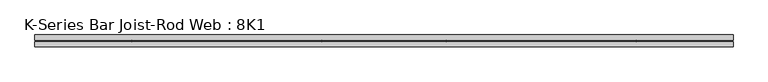
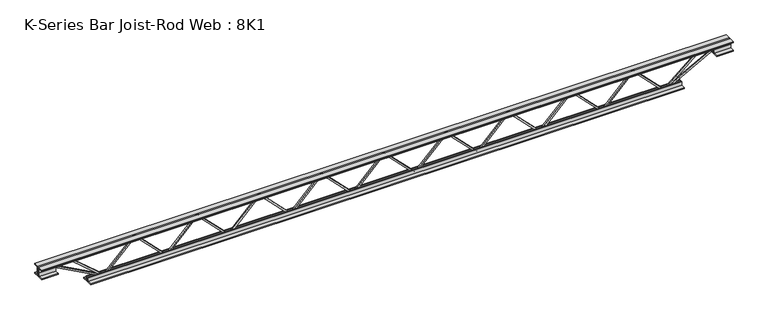
"""IFC4 building model written with IfcOpenShell, lengths in millimetres: beam geometry, K-Series Bar Joist-Rod Web : 8K1."""

import ifcopenshell
import ifcopenshell.guid

model = None  # the IFC model being written
_history = None  # IfcOwnerHistory: only IFC2X3 demands one
_inside = {}  # id of a spatial element -> (the spatial element, [elements in it])
_under = {}  # id of a project, library or spatial element -> (it, [spatial elements below it])
_declared = {}  # id of a project -> (the project, [libraries it declares])
_typed = {}  # id of a type object -> (the type object, [elements of that type])
_made_of = {}  # id of a material, layer set ... -> (it, [elements and type objects made of it])


def new_model(schema):
    """Start an empty IFC model of exactly this schema.

    Asked for "IFC4X3", IfcOpenShell would pick the latest addendum, in which some entities
    have other attributes; the version numbers below select the first issue.
    IFC2X3 requires an IfcOwnerHistory on every rooted entity: one is made here for all.
    """
    global model, _history
    if schema == "IFC4X3":
        model = ifcopenshell.file(schema_version=(4, 3, 0, 0))
    else:
        model = ifcopenshell.file(schema=schema)
    _inside.clear()
    _under.clear()
    _declared.clear()
    _typed.clear()
    _made_of.clear()
    _history = None
    if model.schema == "IFC2X3":
        org = make("IfcOrganization", Name="unknown")
        user = make(
            "IfcPersonAndOrganization",
            ThePerson=make("IfcPerson", FamilyName="unknown"),
            TheOrganization=org,
        )
        app = make(
            "IfcApplication",
            ApplicationDeveloper=org,
            Version="unknown",
            ApplicationFullName="unknown",
            ApplicationIdentifier="unknown",
        )
        _history = make(
            "IfcOwnerHistory",
            OwningUser=user,
            OwningApplication=app,
            ChangeAction="ADDED",
            CreationDate=0,
        )
    return model


def make(cls, **values):
    """One entity of the class cls with the attributes given. An attribute that is None is left unset."""
    return model.create_entity(
        cls, **{name: value for name, value in values.items() if value is not None}
    )


def rooted(cls, **values):
    """An entity with a GlobalId (a new one), such as an element, a storey or a relation."""
    return make(cls, GlobalId=ifcopenshell.guid.new(), OwnerHistory=_history, **values)


def si_unit(unit_type, name, prefix=None):
    """IfcSIUnit, for example si_unit("LENGTHUNIT", "METRE", prefix="MILLI")."""
    return make("IfcSIUnit", UnitType=unit_type, Prefix=prefix, Name=name)


def assignment(units):
    """IfcUnitAssignment: the units of a project."""
    return None if units is None else make("IfcUnitAssignment", Units=units)


def point(xyz):
    """IfcCartesianPoint."""
    return None if xyz is None else make("IfcCartesianPoint", Coordinates=xyz)


def direction(xyz):
    """IfcDirection."""
    return None if xyz is None else make("IfcDirection", DirectionRatios=xyz)


def frame(location, z_axis=None, x_axis=None):
    """IfcAxis2Placement3D, a coordinate frame: its origin and axes. An axis left out is left unset."""
    return make(
        "IfcAxis2Placement3D",
        Location=point(location),
        Axis=direction(z_axis),
        RefDirection=direction(x_axis),
    )


def origin():
    """The frame at (0, 0, 0) with its axes left unset."""
    return frame((0.0, 0.0, 0.0))


def place(relative_to, where):
    """IfcLocalPlacement: puts the frame where relative to a parent placement (None: the world)."""
    return make(
        "IfcLocalPlacement", PlacementRelTo=relative_to, RelativePlacement=where
    )


def context(
    kind, dimensions, precision=None, world=None, true_north=None, identifier=None
):
    """IfcGeometricRepresentationContext, for example the 3D "Model" context."""
    return make(
        "IfcGeometricRepresentationContext",
        ContextIdentifier=identifier,
        ContextType=kind,
        CoordinateSpaceDimension=dimensions,
        Precision=precision,
        WorldCoordinateSystem=world,
        TrueNorth=true_north,
    )


def project(units=None, contexts=None):
    """IfcProject with its units and contexts."""
    return rooted(
        "IfcProject",
        Name="project",
        RepresentationContexts=contexts,
        UnitsInContext=assignment(units),
    )


def spatial(cls, under=None, at=None, **own):
    """A site, building, storey or space (cls), placed at a placement, below another one or the project."""
    s = rooted(cls, ObjectPlacement=at, **own)
    if under is not None:
        _under.setdefault(under.id(), (under, []))[1].append(s)
    return s


def polyline(points):
    """IfcPolyline through the points."""
    return make("IfcPolyline", Points=[point(p) for p in points])


def outline(outer, holes=None, kind="AREA"):
    """IfcArbitraryClosedProfileDef: a profile drawn as a closed curve; with holes, ...WithVoids."""
    if holes is None:
        return make("IfcArbitraryClosedProfileDef", ProfileType=kind, OuterCurve=outer)
    return make(
        "IfcArbitraryProfileDefWithVoids",
        ProfileType=kind,
        OuterCurve=outer,
        InnerCurves=holes,
    )


def extrude(swept, where, along, depth):
    """IfcExtrudedAreaSolid: the profile swept, set in the frame where, extruded along a direction by depth."""
    return make(
        "IfcExtrudedAreaSolid",
        SweptArea=swept,
        Position=where,
        ExtrudedDirection=direction(along),
        Depth=depth,
    )


def shape(context_of_items, identifier, shape_type, items):
    """IfcShapeRepresentation: the items that make up one representation, for example the "Body"."""
    return make(
        "IfcShapeRepresentation",
        ContextOfItems=context_of_items,
        RepresentationIdentifier=identifier,
        RepresentationType=shape_type,
        Items=items,
    )


def source(mapping_origin, context_of_items, identifier, shape_type, items):
    """IfcRepresentationMap: a shape defined once, which mapped items show again and again."""
    return make(
        "IfcRepresentationMap",
        MappingOrigin=mapping_origin,
        MappedRepresentation=shape(context_of_items, identifier, shape_type, items),
    )


def transform(
    local_origin,
    x_axis=None,
    y_axis=None,
    z_axis=None,
    scale=None,
    scale2=None,
    scale3=None,
    uniform=True,
):
    """IfcCartesianTransformationOperator3D, or its non-uniform kind. x_axis, y_axis, z_axis: its Axis1, 2, 3."""
    if uniform:
        return make(
            "IfcCartesianTransformationOperator3D",
            Axis1=direction(x_axis),
            Axis2=direction(y_axis),
            LocalOrigin=point(local_origin),
            Scale=scale,
            Axis3=direction(z_axis),
        )
    return make(
        "IfcCartesianTransformationOperator3DnonUniform",
        Axis1=direction(x_axis),
        Axis2=direction(y_axis),
        LocalOrigin=point(local_origin),
        Scale=scale,
        Axis3=direction(z_axis),
        Scale2=scale2,
        Scale3=scale3,
    )


def mapped(mapping_source, mapping_target):
    """IfcMappedItem: shows the shape of a source again, moved by a transform."""
    return make(
        "IfcMappedItem", MappingSource=mapping_source, MappingTarget=mapping_target
    )


def made_of(thing, what):
    """Note that an element or type object is made of a material, layer set ...; save() writes the relation."""
    if what is not None:
        _made_of.setdefault(what.id(), (what, []))[1].append(thing)
    return thing


def element(
    cls,
    number,
    at=None,
    inside=None,
    cuts=None,
    type_object=None,
    material=None,
    context=None,
    identifier="Body",
    shape_type=None,
    held_by="IfcProductDefinitionShape",
    body=None,
    shapes=None,
    **own,
):
    """One element of the class cls, such as IfcWall. Its Tag is "e" and its number.

    at: its placement. inside: the storey or other place that contains it. cuts: it is an
    opening in that element (IfcRelVoidsElement). A single representation is given by context,
    identifier, shape_type and body (its items); several are given by shapes. held_by: the class
    of the entity that holds the representations. save() writes the other relations.
    """
    e = rooted(cls, Tag="e%d" % number, ObjectPlacement=at, **own)
    if body is not None:
        shapes = [shape(context, identifier, shape_type, body)]
    if shapes is not None:
        e.Representation = make(held_by, Representations=shapes)
    if inside is not None:
        _inside.setdefault(inside.id(), (inside, []))[1].append(e)
    if cuts is not None:
        rooted(
            "IfcRelVoidsElement", RelatingBuildingElement=cuts, RelatedOpeningElement=e
        )
    if type_object is not None:
        _typed.setdefault(type_object.id(), (type_object, []))[1].append(e)
    return made_of(e, material)


def aggregate(whole, parts):
    """IfcRelAggregates: a whole, such as a stair, and the parts it consists of."""
    return rooted("IfcRelAggregates", RelatingObject=whole, RelatedObjects=parts)


def save(model, path):
    """Write the relations noted so far, then the file.

    IfcRelAggregates (storeys below a building ...), IfcRelContainedInSpatialStructure (elements
    in a storey), IfcRelDefinesByType, IfcRelAssociatesMaterial and IfcRelDeclares: one each for
    every whole, place, type object, material and project.
    """
    for whole, parts in _under.values():
        aggregate(whole, parts)
    for where, things in _inside.values():
        rooted(
            "IfcRelContainedInSpatialStructure",
            RelatedElements=things,
            RelatingStructure=where,
        )
    for kind, things in _typed.values():
        rooted("IfcRelDefinesByType", RelatedObjects=things, RelatingType=kind)
    for what, things in _made_of.values():
        rooted("IfcRelAssociatesMaterial", RelatedObjects=things, RelatingMaterial=what)
    for by, libraries in _declared.values():
        rooted("IfcRelDeclares", RelatingContext=by, RelatedDefinitions=libraries)
    model.write(path)


def k_series_bar_joist_rod_web_8k1_4aadf061(model_context):
    return source(origin(), model_context, "Body", "SweptSolid", [
        extrude(outline(polyline([(-90.4875, 968.3504289), (-100.0125, 968.3504289), (-100.0125, 973.521642), (90.4875, 1160.8417278), (90.4875, 1163.1993017), (-100.0125, 1350.5193875), (-100.0125, 1355.6906005), (-90.4875, 1355.6906005), (-90.4875, 1354.5118136), (100.0125, 1167.1917278), (100.0125, 1156.8493017), (-90.4875, 969.5292159), (-90.4875, 968.3504289)])), frame((0.0, -4.7625, 0.0), z_axis=(0.0, 1.0, 0.0), x_axis=(0.0, 0.0, 1.0)), (0.0, 0.0, 1.0), 9.525),
        extrude(outline(polyline([(-90.4875, 581.0102574), (-100.0125, 581.0102574), (-100.0125, 586.1814704), (90.4875, 773.5015562), (90.4875, 775.8591301), (-100.0125, 963.1792159), (-100.0125, 968.3504289), (-90.4875, 968.3504289), (-90.4875, 967.171642), (100.0125, 779.8515562), (100.0125, 769.5091301), (-90.4875, 582.1890443), (-90.4875, 581.0102574)])), frame((0.0, -4.7625, 0.0), z_axis=(0.0, 1.0, 0.0), x_axis=(0.0, 0.0, 1.0)), (0.0, 0.0, 1.0), 9.525),
        extrude(outline(polyline([(-90.4875, 193.6700858), (-100.0125, 193.6700858), (-100.0125, 198.8412988), (90.4875, 386.1613846), (90.4875, 388.5189586), (-100.0125, 575.8390443), (-100.0125, 581.0102574), (-90.4875, 581.0102574), (-90.4875, 579.8314704), (100.0125, 392.5113846), (100.0125, 382.1689586), (-90.4875, 194.8488728), (-90.4875, 193.6700858)])), frame((0.0, -4.7625, 0.0), z_axis=(0.0, 1.0, 0.0), x_axis=(0.0, 0.0, 1.0)), (0.0, 0.0, 1.0), 9.525),
        extrude(outline(polyline([(-90.4875, -193.6700858), (-100.0125, -193.6700858), (-100.0125, -188.4988728), (90.4875, -1.178787), (90.4875, 1.178787), (-100.0125, 188.4988728), (-100.0125, 193.6700858), (-90.4875, 193.6700858), (-90.4875, 192.4912988), (100.0125, 5.171213), (100.0125, -5.171213), (-90.4875, -192.4912988), (-90.4875, -193.6700858)])), frame((0.0, -4.7625, 0.0), z_axis=(0.0, 1.0, 0.0), x_axis=(0.0, 0.0, 1.0)), (0.0, 0.0, 1.0), 9.525),
        extrude(outline(polyline([(-90.4875, -581.0102574), (-100.0125, -581.0102574), (-100.0125, -575.8390443), (90.4875, -388.5189586), (90.4875, -386.1613846), (-100.0125, -198.8412988), (-100.0125, -193.6700858), (-90.4875, -193.6700858), (-90.4875, -194.8488728), (100.0125, -382.1689586), (100.0125, -392.5113846), (-90.4875, -579.8314704), (-90.4875, -581.0102574)])), frame((0.0, -4.7625, 0.0), z_axis=(0.0, 1.0, 0.0), x_axis=(0.0, 0.0, 1.0)), (0.0, 0.0, 1.0), 9.525),
        extrude(outline(polyline([(-90.4875, -968.3504289), (-100.0125, -968.3504289), (-100.0125, -963.1792159), (90.4875, -775.8591301), (90.4875, -773.5015562), (-100.0125, -586.1814704), (-100.0125, -581.0102574), (-90.4875, -581.0102574), (-90.4875, -582.1890443), (100.0125, -769.5091301), (100.0125, -779.8515562), (-90.4875, -967.171642), (-90.4875, -968.3504289)])), frame((0.0, -4.7625, 0.0), z_axis=(0.0, 1.0, 0.0), x_axis=(0.0, 0.0, 1.0)), (0.0, 0.0, 1.0), 9.525),
        extrude(outline(polyline([(-90.4875, -1355.6906005), (-100.0125, -1355.6906005), (-100.0125, -1350.5193875), (90.4875, -1163.1993017), (90.4875, -1160.8417278), (-100.0125, -973.521642), (-100.0125, -968.3504289), (-90.4875, -968.3504289), (-90.4875, -969.5292159), (100.0125, -1156.8493017), (100.0125, -1167.1917278), (-90.4875, -1354.5118136), (-90.4875, -1355.6906005)])), frame((0.0, -4.7625, 0.0), z_axis=(0.0, 1.0, 0.0), x_axis=(0.0, 0.0, 1.0)), (0.0, 0.0, 1.0), 9.525),
        extrude(outline(polyline([(-90.4875, 1355.6906005), (-100.0125, 1355.6906005), (-100.0125, 1360.8618136), (90.4875, 1548.1818993), (90.4875, 1550.5394733), (-100.0125, 1737.8595591), (-100.0125, 1743.0307721), (-90.4875, 1743.0307721), (-90.4875, 1741.8519851), (100.0125, 1554.5318993), (100.0125, 1544.1894733), (-90.4875, 1356.8693875), (-90.4875, 1355.6906005)])), frame((0.0, -4.7625, 0.0), z_axis=(0.0, 1.0, 0.0), x_axis=(0.0, 0.0, 1.0)), (0.0, 0.0, 1.0), 9.525),
        extrude(outline(polyline([(-90.4875, -1743.0307721), (-100.0125, -1743.0307721), (-100.0125, -1737.8595591), (90.4875, -1550.5394733), (90.4875, -1548.1818993), (-100.0125, -1360.8618136), (-100.0125, -1355.6906005), (-90.4875, -1355.6906005), (-90.4875, -1356.8693875), (100.0125, -1544.1894733), (100.0125, -1554.5318993), (-90.4875, -1741.8519851), (-90.4875, -1743.0307721)])), frame((0.0, -4.7625, 0.0), z_axis=(0.0, 1.0, 0.0), x_axis=(0.0, 0.0, 1.0)), (0.0, 0.0, 1.0), 9.525),
        extrude(outline(polyline([(4.7625, 101.6), (36.5125, 101.6), (36.5125, 95.25), (11.1125, 95.25), (11.1125, 69.85), (4.7625, 69.85), (4.7625, 101.6)])), frame((-2149.4307721, 0.0, 0.0), z_axis=(1.0, 0.0, 0.0), x_axis=(0.0, 1.0, 0.0)), (0.0, 0.0, 1.0), 4298.8615442),
        extrude(outline(polyline([(-4.7625, 101.6), (-4.7625, 69.85), (-11.1125, 69.85), (-11.1125, 95.25), (-36.5125, 95.25), (-36.5125, 101.6), (-4.7625, 101.6)])), frame((-2149.4307721, 0.0, 0.0), z_axis=(1.0, 0.0, 0.0), x_axis=(0.0, 1.0, 0.0)), (0.0, 0.0, 1.0), 4298.8615442),
        extrude(outline(polyline([(-4.7625, 38.1), (-36.5125, 38.1), (-36.5125, 44.45), (-11.1125, 44.45), (-11.1125, 69.85), (-4.7625, 69.85), (-4.7625, 38.1)])), frame((-2149.4307721, 0.0, 0.0), z_axis=(1.0, 0.0, 0.0), x_axis=(0.0, 1.0, 0.0)), (0.0, 0.0, 1.0), 101.6),
        extrude(outline(polyline([(36.5125, 38.1), (4.7625, 38.1), (4.7625, 69.85), (11.1125, 69.85), (11.1125, 44.45), (36.5125, 44.45), (36.5125, 38.1)])), frame((-2149.4307721, 0.0, 0.0), z_axis=(1.0, 0.0, 0.0), x_axis=(0.0, 1.0, 0.0)), (0.0, 0.0, 1.0), 101.6),
        extrude(outline(polyline([(4.7625, 38.1), (4.7625, 69.85), (11.1125, 69.85), (11.1125, 44.45), (36.5125, 44.45), (36.5125, 38.1), (4.7625, 38.1)])), frame((2047.8307721, 0.0, 0.0), z_axis=(1.0, 0.0, 0.0), x_axis=(0.0, 1.0, 0.0)), (0.0, 0.0, 1.0), 101.6),
        extrude(outline(polyline([(-4.7625, 38.1), (-36.5125, 38.1), (-36.5125, 44.45), (-11.1125, 44.45), (-11.1125, 69.85), (-4.7625, 69.85), (-4.7625, 38.1)])), frame((2047.8307721, 0.0, 0.0), z_axis=(1.0, 0.0, 0.0), x_axis=(0.0, 1.0, 0.0)), (0.0, 0.0, 1.0), 101.6),
        extrude(outline(polyline([(4.7625, -101.6), (4.7625, -69.85), (11.1125, -69.85), (11.1125, -95.25), (36.5125, -95.25), (36.5125, -101.6), (4.7625, -101.6)])), frame((-1844.6307721, 0.0, 0.0), z_axis=(1.0, 0.0, 0.0), x_axis=(0.0, 1.0, 0.0)), (0.0, 0.0, 1.0), 3689.2615442),
        extrude(outline(polyline([(-4.7625, -101.6), (-36.5125, -101.6), (-36.5125, -95.25), (-11.1125, -95.25), (-11.1125, -69.85), (-4.7625, -69.85), (-4.7625, -101.6)])), frame((-1844.6307721, 0.0, 0.0), z_axis=(1.0, 0.0, 0.0), x_axis=(0.0, 1.0, 0.0)), (0.0, 0.0, 1.0), 3689.2615442),
        extrude(outline(polyline([(0.0, -9.525), (0.0, 0.0), (346.6425392, 0.0), (346.6425392, -9.525), (0.0, -9.525)])), frame((-2050.0990706, 4.7625, 65.662372), z_axis=(0.47628314854008014, 0.0, 0.8792919665371384), x_axis=(0.8792919665371384, 0.0, -0.47628314854008014)), (0.0, 0.0, 1.0), 9.525),
        extrude(outline(polyline([(0.0, -9.525), (0.0, 0.0), (254.4918705, 0.0), (254.4918705, -9.525), (0.0, -9.525)])), frame((-1939.7904998, 4.7625, 66.2257043), z_axis=(0.6487437091878946, 0.0, 0.7610069643499542), x_axis=(0.7610069643499542, 0.0, -0.6487437091878946)), (0.0, 0.0, 1.0), 9.525),
        extrude(outline(polyline([(0.0, -9.525), (0.0, 0.0), (346.6425392, 0.0), (346.6425392, -9.525), (0.0, -9.525)])), frame((2050.0990706, -4.7625, 65.662372), z_axis=(-0.476283148540043, 0.0, 0.8792919665371586), x_axis=(-0.8792919665371586, 0.0, -0.476283148540043)), (0.0, 0.0, 1.0), 9.525),
        extrude(outline(polyline([(0.0, -9.525), (0.0, 0.0), (254.4918705, 0.0), (254.4918705, -9.525), (0.0, -9.525)])), frame((1939.7904998, -4.7625, 66.2257043), z_axis=(-0.648743709187867, 0.0, 0.7610069643499777), x_axis=(-0.7610069643499777, 0.0, -0.648743709187867)), (0.0, 0.0, 1.0), 9.525),
    ])


if __name__ == "__main__":
    model = new_model("IFC4")
    model_context = context("Model", 3, world=origin())
    ifc_project = project(units=[si_unit("LENGTHUNIT", "METRE", prefix="MILLI")], contexts=[model_context])
    site = spatial("IfcSite", under=ifc_project)
    building = spatial("IfcBuilding", under=site)
    placement = place(None, origin())
    k_series_bar_joist_rod_web_8k1_shape = k_series_bar_joist_rod_web_8k1_4aadf061(model_context)
    element("IfcBeam", 1, ObjectType="K-Series Bar Joist-Rod Web : 8K1", at=placement, inside=building, context=model_context, shape_type="MappedRepresentation", body=[
        mapped(k_series_bar_joist_rod_web_8k1_shape, transform((0.0, 0.0, 0.0), x_axis=(1.0, 0.0, 0.0), y_axis=(0.0, 1.0, 0.0), z_axis=(0.0, 0.0, 1.0))),
    ])
    save(model, "model.ifc")

# Revit data of these elements
# Type "K-Series Bar Joist-Rod Web : 8K1"
#   Assembly Code = "B1010350"
#   Wt = 5.1
#   Web Thickness = 0' - 0 3/8"
#   Start Offset [instance default] = 0' - 0"
#   Start Extension [instance default] = 0' - 0"
#   Seat Length = 0' - 4"
#   Seat Depth = 0' - 2 1/2"
#   PanelArrayLength [instance default] = 21' - 4"
#   Panel [instance default] = 1' - 4"
#   End Offset [instance default] = 0' - 0"
#   End Extension [instance default] = 0' - 0"
#   End Panel = 1' - 4"
#   Cord Leg = 0' - 1 1/4"
#   Chord Thickness = 0' - 0 1/4"
#   Length [instance default] = 24' - 0"
#   Depth = 0' - 8"
#   PanelArrayNum [instance default] = 16
#   Rendering Material = none
# Element 1 (IfcBeam, "K-Series Bar Joist-Rod Web : 8K1")
#   PanelArrayLength = 11' - 5.24652"
#   Panel = 1' - 3.24961"
#   PanelArrayNum = 9
